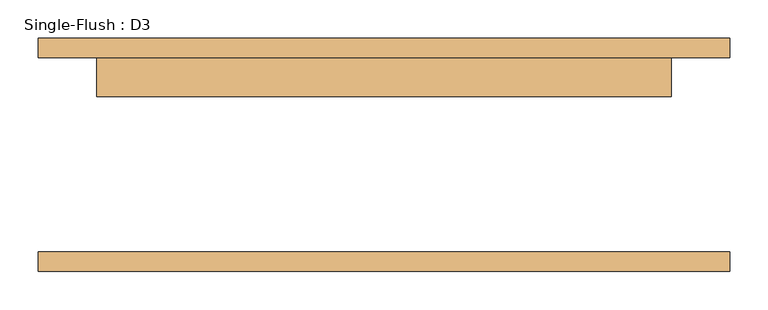
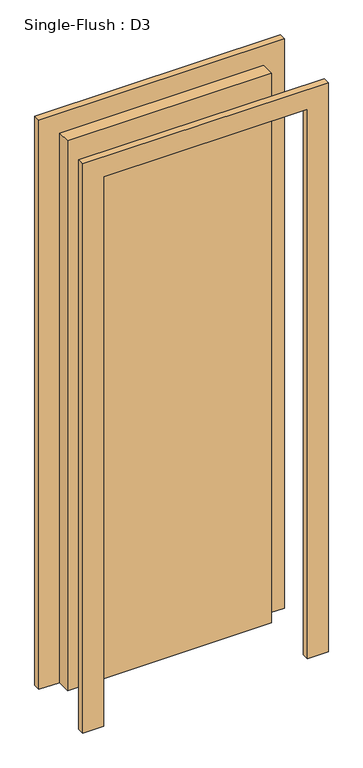
"""IFC4 building model written with IfcOpenShell, lengths in millimetres: door geometry, Single-Flush : D3."""

from ifc_helpers import new_model, si_unit, frame, origin, origin_with_axes, place, context, project, spatial, polyline, outline, extrude, source, transform, mapped, element, save


def single_flush_d3_8acf0758(model_context):
    return source(origin(), model_context, "Body", "SweptSolid", [
        extrude(outline(polyline([(2209.8, -451.2), (0.0, -451.2), (0.0, -375.0), (2133.6, -375.0), (2133.6, 375.0), (0.0, 375.0), (0.0, 451.2), (2209.8, 451.2), (2209.8, -451.2)])), frame((0.0, 127.0, 0.0), z_axis=(0.0, 1.0, 0.0), x_axis=(0.0, 0.0, 1.0)), (0.0, 0.0, 1.0), 25.4),
        extrude(outline(polyline([(2209.8, 451.2), (2209.8, -451.2), (0.0, -451.2), (0.0, -375.0), (2133.6, -375.0), (2133.6, 375.0), (0.0, 375.0), (0.0, 451.2), (2209.8, 451.2)])), frame((0.0, -152.4, 0.0), z_axis=(0.0, 1.0, 0.0), x_axis=(0.0, 0.0, 1.0)), (0.0, 0.0, 1.0), 25.4),
        extrude(outline(polyline([(375.0, 76.2), (-375.0, 76.2), (-375.0, 127.0), (375.0, 127.0), (375.0, 76.2)])), origin_with_axes(), (0.0, 0.0, 1.0), 2133.6),
    ])


if __name__ == "__main__":
    model = new_model("IFC4")
    model_context = context("Model", 3, world=origin())
    ifc_project = project(units=[si_unit("LENGTHUNIT", "METRE", prefix="MILLI")], contexts=[model_context])
    site = spatial("IfcSite", under=ifc_project)
    building = spatial("IfcBuilding", under=site)
    placement = place(None, origin())
    single_flush_d3_shape = single_flush_d3_8acf0758(model_context)
    element("IfcDoor", 1, ObjectType="Single-Flush : D3", at=placement, inside=building, context=model_context, shape_type="MappedRepresentation", body=[
        mapped(single_flush_d3_shape, transform((0.0, 0.0, 0.0), x_axis=(1.0, 0.0, 0.0), y_axis=(0.0, 1.0, 0.0), z_axis=(0.0, 0.0, 1.0))),
    ])
    save(model, "model.ifc")

# Revit data of these elements
# Type "Single-Flush : D3"
#   Type Mark = "D2"
#   Construction Type Id = "MDOOR"
#   Assembly Code = "C1020"
#   Analytic Construction = "Metal"
#   Thickness = 50.8 mm
#   Heat Transfer Coefficient (U) = 3.7021 W/(m²·K)
#   Height = 2133.6 mm
#   Trim Projection Ext = 25.4 mm
#   Trim Projection Int = 25.4 mm
#   Trim Width = 76.2 mm
#   Width = 750 mm
#   Door Material = Door - Panel
#   Frame Material = Door - Frame
#   Visual Light Transmittance = 0
#   Solar Heat Gain Coefficient = 0
#   Function = (empty or 0)
#   Wall Closure = (empty or 0)
# Element 1 (IfcDoor, "Single-Flush : D3")
#   Materials on its faces: "Door - Frame", "Door - Panel"
# Materials
#   "Door - Panel": class "Wood", colour RGB 210 159 95, transparency 0
#   "Door - Frame": class "Miscellaneous", colour RGB 118 70 51, transparency 0
